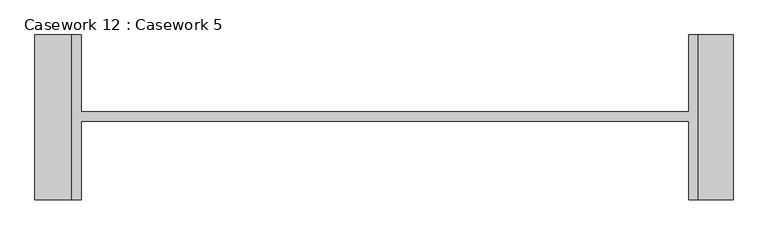
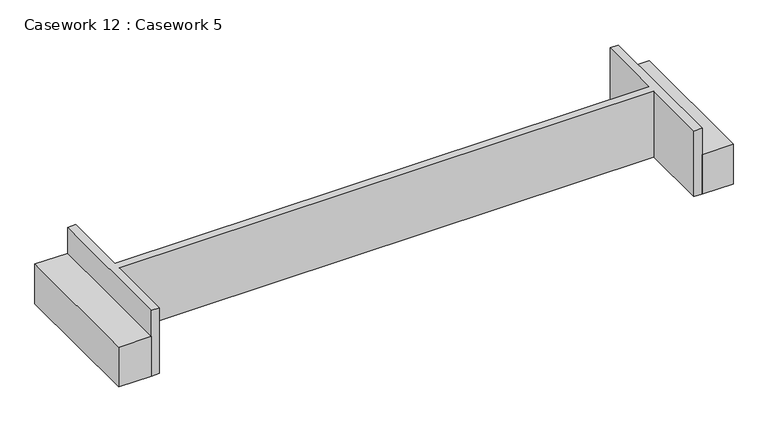
"""IFC4 building model written with IfcOpenShell, lengths in millimetres: furniture geometry, Casework 12 : Casework 5."""

from ifc_helpers import new_model, si_unit, origin, origin_with_axes, place, context, project, spatial, polyline, outline, extrude, source, transform, mapped, element, save


def casework_12_casework_5_d3ae8625(model_context):
    return source(origin(), model_context, "Body", "SweptSolid", [
        extrude(outline(polyline([(-45222.23615, 263718.5701927), (-45222.23615, 261177.5188832), (-45765.6431786, 261177.5188832), (-45765.6431786, 263718.5701927), (-45222.23615, 263718.5701927)])), origin_with_axes(), (0.0, 0.0, 1.0), 736.6),
        extrude(outline(polyline([(-55407.3218514, 263718.5701927), (-55407.3218514, 261177.5188832), (-55978.0010565, 261177.5188832), (-55978.0010565, 263718.5701927), (-55407.3218514, 263718.5701927)])), origin_with_axes(), (0.0, 0.0, 1.0), 736.6),
        extrude(outline(polyline([(-55264.4443999, 263718.5701927), (-55264.4443999, 262531.3616783), (-45907.3606126, 262531.3616783), (-45907.3606126, 263718.5701927), (-45765.6431786, 263718.5701927), (-45765.6431786, 261177.5188832), (-45907.3606126, 261177.5188832), (-45907.3606126, 262389.4983598), (-55264.4443999, 262389.4983598), (-55264.4443999, 261177.5188832), (-55407.3218514, 261177.5188832), (-55407.3218514, 263718.5701927), (-55264.4443999, 263718.5701927)])), origin_with_axes(), (0.0, 0.0, 1.0), 1219.2),
    ])


if __name__ == "__main__":
    model = new_model("IFC4")
    model_context = context("Model", 3, world=origin())
    ifc_project = project(units=[si_unit("LENGTHUNIT", "METRE", prefix="MILLI")], contexts=[model_context])
    site = spatial("IfcSite", under=ifc_project)
    building = spatial("IfcBuilding", under=site)
    placement = place(None, origin())
    casework_12_casework_5_shape = casework_12_casework_5_d3ae8625(model_context)
    element("IfcFurniture", 1, ObjectType="Casework 12 : Casework 5", at=placement, inside=building, context=model_context, shape_type="MappedRepresentation", body=[
        mapped(casework_12_casework_5_shape, transform((0.0, 0.0, 0.0), x_axis=(1.0, 0.0, 0.0), y_axis=(0.0, 1.0, 0.0), z_axis=(0.0, 0.0, 1.0))),
    ])
    save(model, "model.ifc")

# Revit data of these elements
# Element 1 (IfcFurniture, "Casework 12 : Casework 5")
#   Materials on its faces: "WOOD VENEER"
# Materials
#   "WOOD VENEER": class "Miscellaneous", colour RGB 164 164 164, transparency 0, Cost = 0
